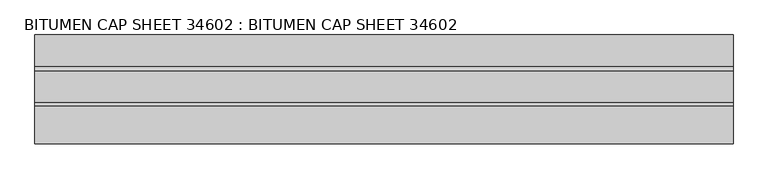
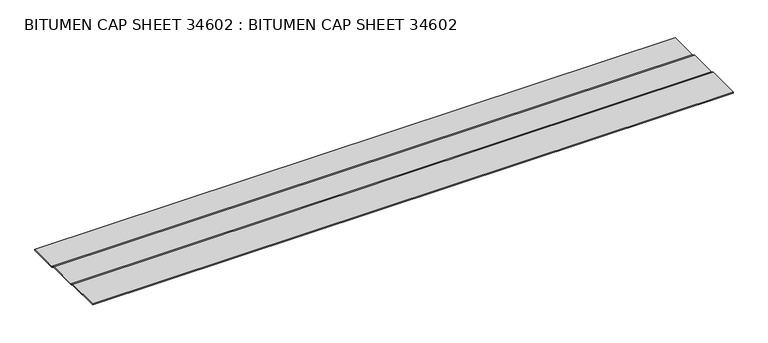
"""IFC4 building model written with IfcOpenShell, lengths in millimetres: proxy geometry, BITUMEN CAP SHEET 34602 : BITUMEN CAP SHEET 34602."""

from ifc_helpers import new_model, si_unit, frame, origin, place, context, project, spatial, polyline, outline, extrude, source, transform, mapped, element, save


def bitumen_cap_sheet_34602_bitumen_cap_sheet_34602_a55ad838(model_context):
    return source(origin(), model_context, "Body", "SweptSolid", [
        extrude(outline(polyline([(-5237.2758356, 40238.7580714), (-5329.4404972, 40238.7580714), (-5341.9053158, 40244.0440809), (-5432.619472, 40244.0440809), (-5442.3358585, 40248.3766459), (-5549.5470696, 40248.3766459), (-5549.5470696, 40251.5518755), (-5441.660573, 40251.5518755), (-5431.9436715, 40247.2190809), (-5341.2599159, 40247.2190809), (-5328.7950972, 40241.9330714), (-5237.2758356, 40241.9330714), (-5237.2758356, 40238.7580714)])), frame((12382.7678845, 0.0, 0.0), z_axis=(1.0, 0.0, 0.0), x_axis=(0.0, 1.0, 0.0)), (0.0, 0.0, 1.0), 2000.25),
    ])


if __name__ == "__main__":
    model = new_model("IFC4")
    model_context = context("Model", 3, world=origin())
    ifc_project = project(units=[si_unit("LENGTHUNIT", "METRE", prefix="MILLI")], contexts=[model_context])
    site = spatial("IfcSite", under=ifc_project)
    building = spatial("IfcBuilding", under=site)
    placement = place(None, origin())
    bitumen_cap_sheet_34602_bitumen_cap_sheet_34602_shape = bitumen_cap_sheet_34602_bitumen_cap_sheet_34602_a55ad838(model_context)
    element("IfcBuildingElementProxy", 1, Name="BITUMEN CAP SHEET 34602 : BITUMEN CAP SHEET 34602", ObjectType="BITUMEN CAP SHEET 34602 : BITUMEN CAP SHEET 34602", at=placement, inside=building, context=model_context, shape_type="MappedRepresentation", body=[
        mapped(bitumen_cap_sheet_34602_bitumen_cap_sheet_34602_shape, transform((0.0, 0.0, 0.0), x_axis=(1.0, 0.0, 0.0), y_axis=(0.0, 1.0, 0.0), z_axis=(0.0, 0.0, 1.0))),
    ])
    save(model, "model.ifc")

# Revit data of these elements
# Type "BITUMEN CAP SHEET 34602 : BITUMEN CAP SHEET 34602"
#   NameOverride = "BITUMEN CAP SHEET"
# Element 1 (IfcBuildingElementProxy, "BITUMEN CAP SHEET 34602 : BITUMEN CAP SHEET 34602")
#   Materials on its faces: "MODIFIED BITUMEN GRANULE SURFACED CAP SHEET"
# Materials
#   "MODIFIED BITUMEN GRANULE SURFACED CAP SHEET": class "Unassigned", colour RGB 85 85 127, transparency 0
